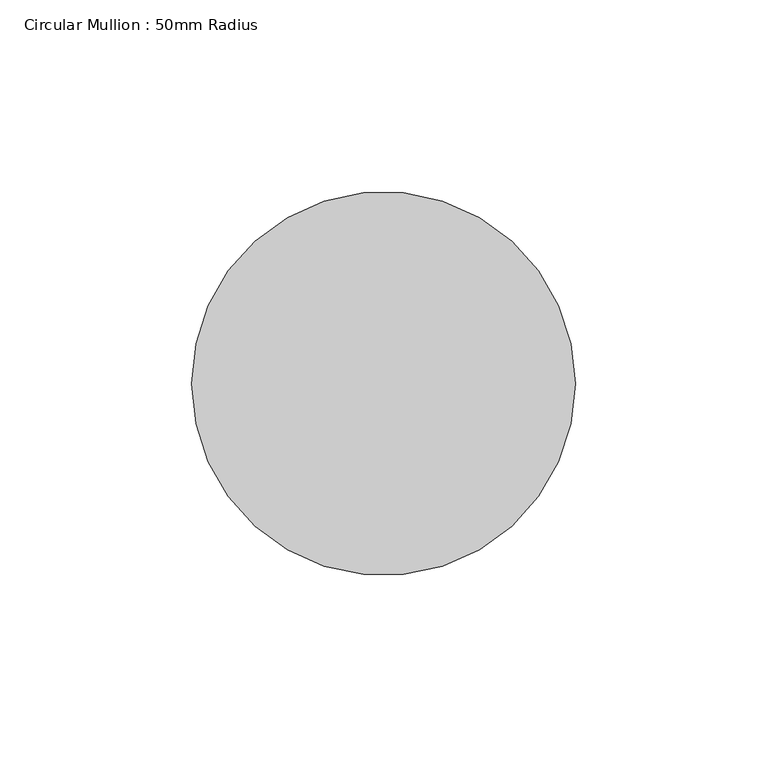
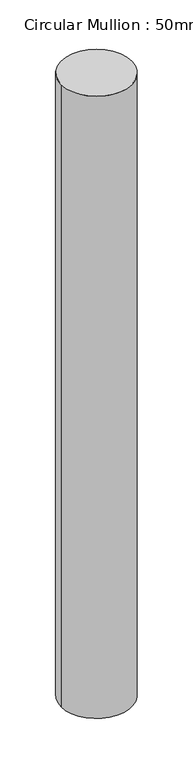
"""IFC4 building model written with IfcOpenShell, lengths in millimetres: member geometry, Circular Mullion : 50mm Radius."""

from ifc_helpers import new_model, si_unit, point, frame, origin, origin_2d, place, context, project, spatial, circle_curve, trimmed, segment, composite_curve, outline, extrude, source, transform, mapped, element, save


def circular_mullion_50mm_radius_3c98ecd6(model_context):
    return source(origin(), model_context, "Body", "SweptSolid", [
        extrude(outline(composite_curve([segment(trimmed(circle_curve(origin_2d(), 50.0), [point((50.0, 0.0))], [point((-50.0, 0.0))], False, "CARTESIAN"), True, "CONTINUOUS"), segment(trimmed(circle_curve(origin_2d(), 50.0), [point((-50.0, 0.0))], [point((50.0, 0.0))], False, "CARTESIAN"), True, "CONTINUOUS")], self_intersect=False)), frame((0.0, 0.0, -929.1777459), z_axis=(0.0, 0.0, 1.0), x_axis=(1.0, 0.0, 0.0)), (0.0, 0.0, 1.0), 929.1777459),
    ])


if __name__ == "__main__":
    model = new_model("IFC4")
    model_context = context("Model", 3, world=origin())
    ifc_project = project(units=[si_unit("LENGTHUNIT", "METRE", prefix="MILLI")], contexts=[model_context])
    site = spatial("IfcSite", under=ifc_project)
    building = spatial("IfcBuilding", under=site)
    placement = place(None, origin())
    circular_mullion_50mm_radius_shape = circular_mullion_50mm_radius_3c98ecd6(model_context)
    element("IfcMember", 1, ObjectType="Circular Mullion : 50mm Radius", at=placement, inside=building, context=model_context, shape_type="MappedRepresentation", body=[
        mapped(circular_mullion_50mm_radius_shape, transform((0.0, 0.0, 0.0), x_axis=(1.0, 0.0, 0.0), y_axis=(0.0, 1.0, 0.0), z_axis=(0.0, 0.0, 1.0))),
    ])
    save(model, "model.ifc")

# Revit data of these elements
# Type "Circular Mullion : 50mm Radius"
#   built-in parameter 1007350 = 0.164042 (stored number, unit not read)
# Element 1 (IfcMember, "Circular Mullion : 50mm Radius")
#   Materials on its faces: "Aluminium"
# Materials
#   "Aluminium": class "Metal", colour RGB 247 247 247, transparency 0, Description = "Aluminium 6061", Cost = 0
